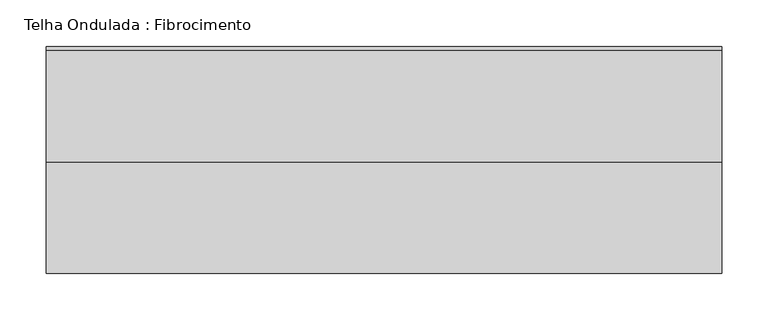
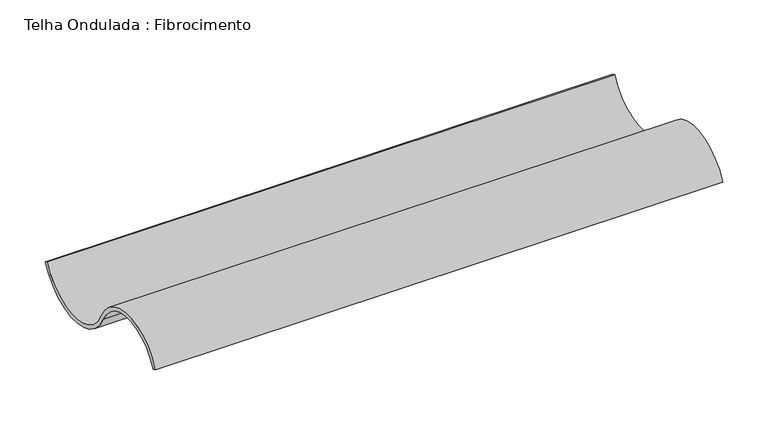
"""IFC4 building model written with IfcOpenShell, lengths in millimetres: beam geometry, Telha Ondulada : Fibrocimento."""

from ifc_helpers import new_model, si_unit, point, frame, frame_2d, origin, place, context, project, spatial, polyline, circle_curve, trimmed, segment, composite_curve, outline, extrude, source, transform, mapped, element, save


def telha_ondulada_fibrocimento_963230a9(model_context):
    return source(origin(), model_context, "Body", "SweptSolid", [
        extrude(outline(composite_curve([segment(trimmed(circle_curve(frame_2d((68.3970135, 71.7939461)), 66.7939461), [point((8.3970135, 42.4437972))], [point((128.3970135, 42.4437972))], True, "CARTESIAN"), True, "CONTINUOUS"), segment(polyline([(128.3970135, 42.4437972), (132.8884385, 40.2467307)]), True, "CONTINUOUS"), segment(trimmed(circle_curve(frame_2d((68.3970135, 71.7939461)), 71.7939461), [point((132.8884385, 40.2467307))], [point((3.9055884, 40.2467307))], False, "CARTESIAN"), True, "CONTINUOUS"), segment(trimmed(circle_curve(frame_2d((-51.6029865, 13.0936483)), 61.7939461), [point((3.9055884, 40.2467307))], [point((-107.1115615, 40.2467307))], True, "CARTESIAN"), True, "CONTINUOUS"), segment(polyline([(-107.1115615, 40.2467307), (-111.6029865, 42.4437972)]), True, "CONTINUOUS"), segment(trimmed(circle_curve(frame_2d((-51.6029865, 13.0936483)), 66.7939461), [point((-111.6029865, 42.4437972))], [point((8.3970135, 42.4437972))], False, "CARTESIAN"), True, "CONTINUOUS")], self_intersect=False)), frame((-362.9289365, 0.0, 0.0), z_axis=(1.0, 0.0, 0.0), x_axis=(0.0, 1.0, 0.0)), (0.0, 0.0, 1.0), 725.8578731),
    ])


if __name__ == "__main__":
    model = new_model("IFC4")
    model_context = context("Model", 3, world=origin())
    ifc_project = project(units=[si_unit("LENGTHUNIT", "METRE", prefix="MILLI")], contexts=[model_context])
    site = spatial("IfcSite", under=ifc_project)
    building = spatial("IfcBuilding", under=site)
    placement = place(None, origin())
    telha_ondulada_fibrocimento_shape = telha_ondulada_fibrocimento_963230a9(model_context)
    element("IfcBeam", 1, ObjectType="Telha Ondulada : Fibrocimento", at=placement, inside=building, context=model_context, shape_type="MappedRepresentation", body=[
        mapped(telha_ondulada_fibrocimento_shape, transform((0.0, 0.0, 0.0), x_axis=(1.0, 0.0, 0.0), y_axis=(0.0, 1.0, 0.0), z_axis=(0.0, 0.0, 1.0))),
    ])
    save(model, "model.ifc")

# Revit data of these elements
# Type "Telha Ondulada : Fibrocimento"
#   Description = "TELHA ONDULADA FIBROCIMENTO"
#   Cost = 5
#   Length [instance default] = 1.524 m
#   b = 0.07 m
#   h = 0.16 m
#   Structural Material = .TELHA DE FIBROCIMENTO
#   Assembly Code = ""
# Element 1 (IfcBeam, "Telha Ondulada : Fibrocimento")
#   Materials on its faces: ".TELHA DE FIBROCIMENTO"
# Materials
#   ".TELHA DE FIBROCIMENTO": class "CC_TELHADO", colour RGB 77 77 76, transparency 0, Description = "TELHA ONDULADA FIBROCIMENTO", Cost = 0
